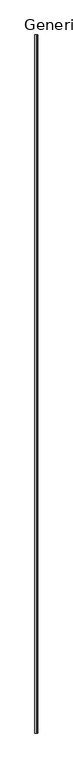
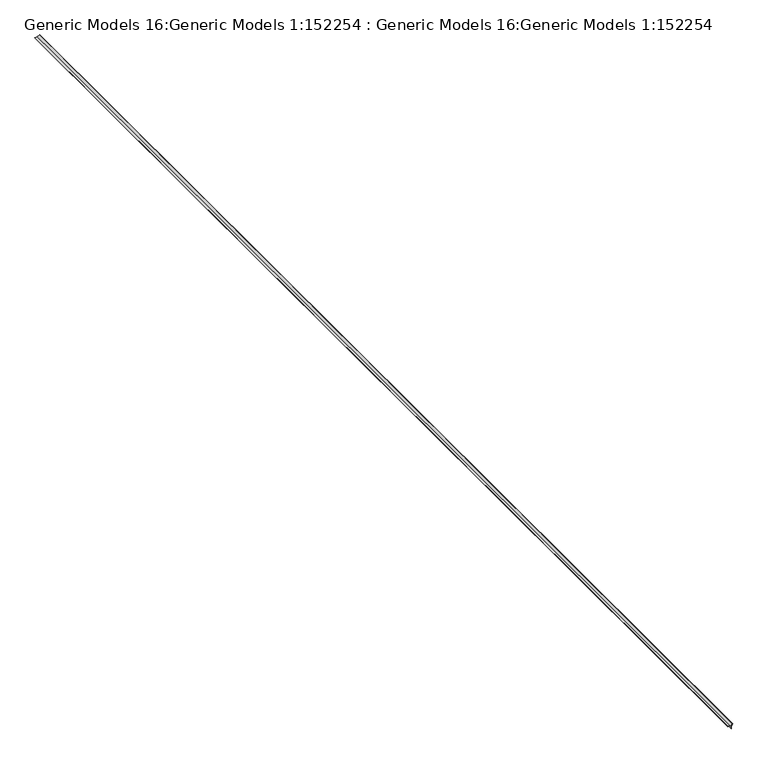
"""IFC4 building model written with IfcOpenShell, lengths in millimetres: proxy geometry, Generic Models 16:Generic Models 1:152254 : Generic Models 16:Generic Models 1:152254."""

from ifc_helpers import new_model, si_unit, point, frame, frame_2d, origin, place, context, project, spatial, polyline, circle_curve, trimmed, segment, composite_curve, outline, extrude, source, transform, mapped, element, save


def generic_models_16_generic_models_1_152254_generic_models_16_94b30d89(model_context):
    return source(origin(), model_context, "Body", "SweptSolid", [
        extrude(outline(composite_curve([segment(trimmed(circle_curve(frame_2d((3651.7491841, -9275.7309996)), 1.4342127), [point((3651.0940291, -9274.4551713))], [point((3653.0250124, -9276.3861547))], False, "CARTESIAN"), True, "CONTINUOUS"), segment(polyline([(3653.0250124, -9276.3861547), (3633.4983968, -9314.4116693), (3633.4983968, -9352.5116693), (3632.2283968, -9352.5116693), (3632.2283968, -9314.1046456), (3652.1286365, -9275.3515473), (3613.3755382, -9295.2517869), (3574.9685144, -9295.2517869), (3574.9685144, -9293.9817869), (3613.0685144, -9293.9817869), (3651.0940291, -9274.4551713)]), True, "CONTINUOUS")], self_intersect=False)), frame((0.0, -6877.9974793, 0.0), z_axis=(0.0, 1.0, 0.0), x_axis=(0.0, 0.0, 1.0)), (0.0, 0.0, 1.0), 19050.0),
    ])


if __name__ == "__main__":
    model = new_model("IFC4")
    model_context = context("Model", 3, world=origin())
    ifc_project = project(units=[si_unit("LENGTHUNIT", "METRE", prefix="MILLI")], contexts=[model_context])
    site = spatial("IfcSite", under=ifc_project)
    building = spatial("IfcBuilding", under=site)
    placement = place(None, origin())
    generic_models_16_generic_models_1_152254_generic_models_16_shape = generic_models_16_generic_models_1_152254_generic_models_16_94b30d89(model_context)
    element("IfcBuildingElementProxy", 1, Name="Generic Models 16:Generic Models 1:152254 : Generic Models 16:Generic Models 1:152254", ObjectType="Generic Models 16:Generic Models 1:152254 : Generic Models 16:Generic Models 1:152254", at=placement, inside=building, context=model_context, shape_type="MappedRepresentation", body=[
        mapped(generic_models_16_generic_models_1_152254_generic_models_16_shape, transform((0.0, 0.0, 0.0), x_axis=(1.0, 0.0, 0.0), y_axis=(0.0, 1.0, 0.0), z_axis=(0.0, 0.0, 1.0))),
    ])
    save(model, "model.ifc")

# Revit data of these elements
# Type "Generic Models 16:Generic Models 1:152254 : Generic Models 16:Generic Models 1:152254"
#   NameOverride = "Generic Models 16:Generic Models 1:152254"
#   ObjectTypeOverride = "Generic Models 16:Generic Models 1"
#   Reference = "Generic Models 1"
#   Category = "Generic Models"
#   Tag = "152254"
# Element 1 (IfcBuildingElementProxy, "Generic Models 16:Generic Models 1:152254 : Generic Models 16:Generic Models 1:152254")
#   Materials on its faces: "_CONTINUOUS 16 GA. COPPER CORNER BEAD 558"
# Materials
#   "_CONTINUOUS 16 GA. COPPER CORNER BEAD 558": class "Unassigned", colour RGB 253 192 103, transparency 0
